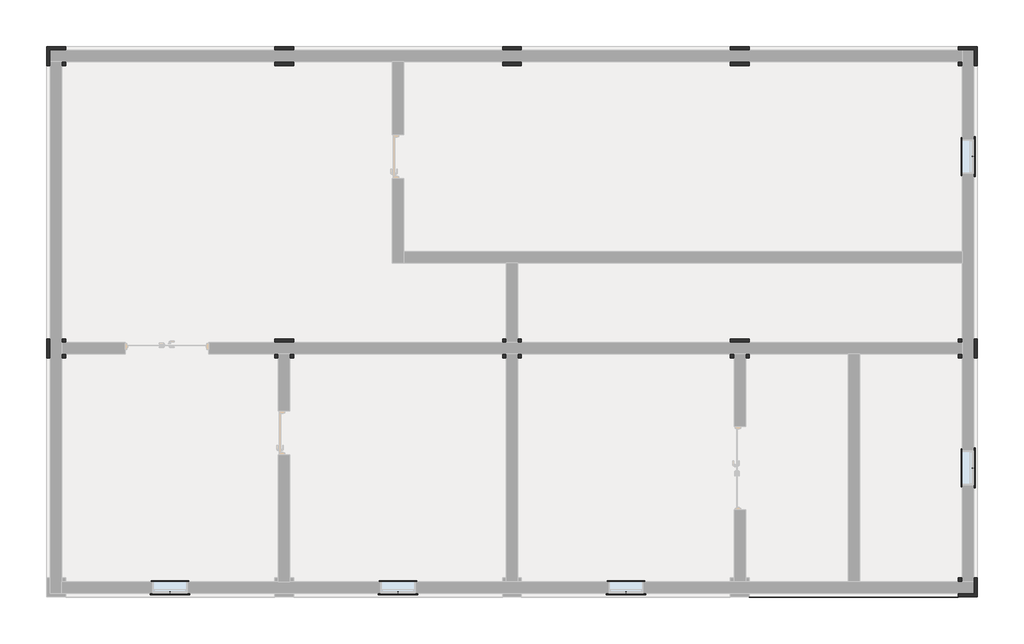
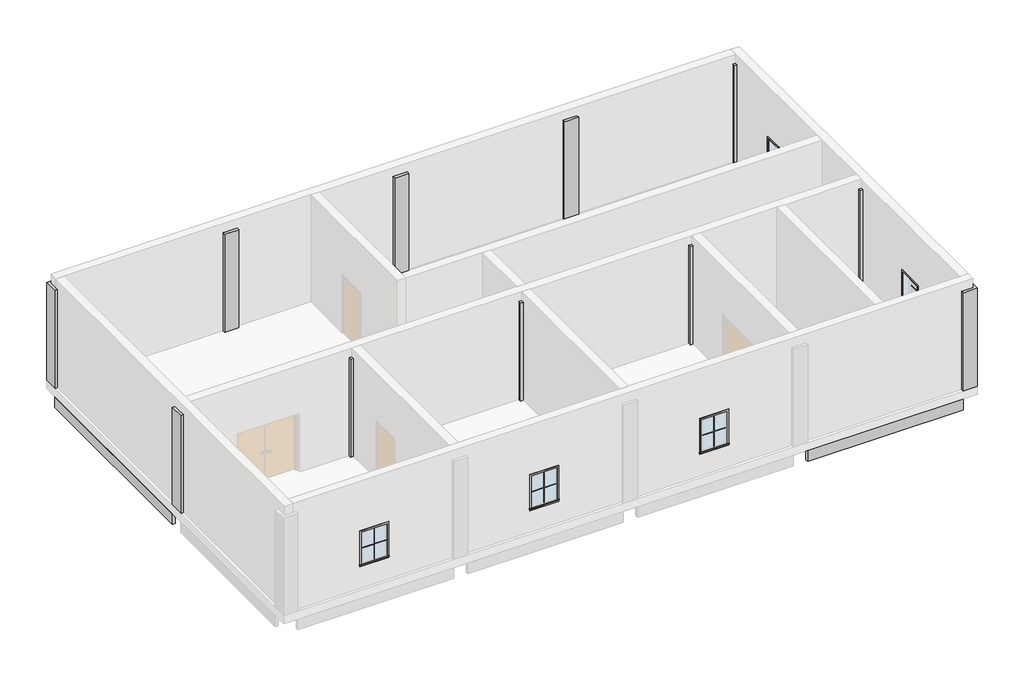
# One storey, part 2 of 2: 16 beams, 15 proxies, 11 columns.
"""IFC4 building model written with IfcOpenShell, lengths in millimetres."""

import ifcopenshell
import ifcopenshell.guid

model = None  # the IFC model being written
_history = None  # IfcOwnerHistory: only IFC2X3 demands one
_inside = {}  # id of a spatial element -> (the spatial element, [elements in it])
_under = {}  # id of a project, library or spatial element -> (it, [spatial elements below it])
_declared = {}  # id of a project -> (the project, [libraries it declares])
_typed = {}  # id of a type object -> (the type object, [elements of that type])
_made_of = {}  # id of a material, layer set ... -> (it, [elements and type objects made of it])


def new_model(schema):
    """Start an empty IFC model of exactly this schema.

    Asked for "IFC4X3", IfcOpenShell would pick the latest addendum, in which some entities
    have other attributes; the version numbers below select the first issue.
    IFC2X3 requires an IfcOwnerHistory on every rooted entity: one is made here for all.
    """
    global model, _history
    if schema == "IFC4X3":
        model = ifcopenshell.file(schema_version=(4, 3, 0, 0))
    else:
        model = ifcopenshell.file(schema=schema)
    _inside.clear()
    _under.clear()
    _declared.clear()
    _typed.clear()
    _made_of.clear()
    _history = None
    if model.schema == "IFC2X3":
        org = make("IfcOrganization", Name="unknown")
        user = make(
            "IfcPersonAndOrganization",
            ThePerson=make("IfcPerson", FamilyName="unknown"),
            TheOrganization=org,
        )
        app = make(
            "IfcApplication",
            ApplicationDeveloper=org,
            Version="unknown",
            ApplicationFullName="unknown",
            ApplicationIdentifier="unknown",
        )
        _history = make(
            "IfcOwnerHistory",
            OwningUser=user,
            OwningApplication=app,
            ChangeAction="ADDED",
            CreationDate=0,
        )
    return model


def make(cls, **values):
    """One entity of the class cls with the attributes given. An attribute that is None is left unset."""
    return model.create_entity(
        cls, **{name: value for name, value in values.items() if value is not None}
    )


def rooted(cls, **values):
    """An entity with a GlobalId (a new one), such as an element, a storey or a relation."""
    return make(cls, GlobalId=ifcopenshell.guid.new(), OwnerHistory=_history, **values)


def si_unit(unit_type, name, prefix=None):
    """IfcSIUnit, for example si_unit("LENGTHUNIT", "METRE", prefix="MILLI")."""
    return make("IfcSIUnit", UnitType=unit_type, Prefix=prefix, Name=name)


def assignment(units):
    """IfcUnitAssignment: the units of a project."""
    return None if units is None else make("IfcUnitAssignment", Units=units)


def point(xyz):
    """IfcCartesianPoint."""
    return None if xyz is None else make("IfcCartesianPoint", Coordinates=xyz)


def direction(xyz):
    """IfcDirection."""
    return None if xyz is None else make("IfcDirection", DirectionRatios=xyz)


def frame(location, z_axis=None, x_axis=None):
    """IfcAxis2Placement3D, a coordinate frame: its origin and axes. An axis left out is left unset."""
    return make(
        "IfcAxis2Placement3D",
        Location=point(location),
        Axis=direction(z_axis),
        RefDirection=direction(x_axis),
    )


def origin():
    """The frame at (0, 0, 0) with its axes left unset."""
    return frame((0.0, 0.0, 0.0))


def origin_with_axes():
    """The frame at (0, 0, 0) with the z axis (0, 0, 1) and the x axis (1, 0, 0) written out."""
    return frame((0.0, 0.0, 0.0), z_axis=(0.0, 0.0, 1.0), x_axis=(1.0, 0.0, 0.0))


def place(relative_to, where):
    """IfcLocalPlacement: puts the frame where relative to a parent placement (None: the world)."""
    return make(
        "IfcLocalPlacement", PlacementRelTo=relative_to, RelativePlacement=where
    )


def context(
    kind, dimensions, precision=None, world=None, true_north=None, identifier=None
):
    """IfcGeometricRepresentationContext, for example the 3D "Model" context."""
    return make(
        "IfcGeometricRepresentationContext",
        ContextIdentifier=identifier,
        ContextType=kind,
        CoordinateSpaceDimension=dimensions,
        Precision=precision,
        WorldCoordinateSystem=world,
        TrueNorth=true_north,
    )


def project(units=None, contexts=None):
    """IfcProject with its units and contexts."""
    return rooted(
        "IfcProject",
        Name="project",
        RepresentationContexts=contexts,
        UnitsInContext=assignment(units),
    )


def spatial(cls, under=None, at=None, **own):
    """A site, building, storey or space (cls), placed at a placement, below another one or the project."""
    s = rooted(cls, ObjectPlacement=at, **own)
    if under is not None:
        _under.setdefault(under.id(), (under, []))[1].append(s)
    return s


def polyline(points):
    """IfcPolyline through the points."""
    return make("IfcPolyline", Points=[point(p) for p in points])


def outline(outer, holes=None, kind="AREA"):
    """IfcArbitraryClosedProfileDef: a profile drawn as a closed curve; with holes, ...WithVoids."""
    if holes is None:
        return make("IfcArbitraryClosedProfileDef", ProfileType=kind, OuterCurve=outer)
    return make(
        "IfcArbitraryProfileDefWithVoids",
        ProfileType=kind,
        OuterCurve=outer,
        InnerCurves=holes,
    )


def extrude(swept, where, along, depth):
    """IfcExtrudedAreaSolid: the profile swept, set in the frame where, extruded along a direction by depth."""
    return make(
        "IfcExtrudedAreaSolid",
        SweptArea=swept,
        Position=where,
        ExtrudedDirection=direction(along),
        Depth=depth,
    )


def faces_of(points, faces, orient=None, outer=None):
    """IfcFace entities. A face is a list of loops; a loop is a list of indices into points, from 0.

    orient and outer hold one flag for each loop. By default every Orientation is true, the
    first loop of a face is its IfcFaceOuterBound and the others are IfcFaceBound.
    """
    made = []
    for i, loops in enumerate(faces):
        bounds = []
        for j, loop in enumerate(loops):
            is_outer = j == 0 if outer is None else outer[i][j]
            bounds.append(
                make(
                    "IfcFaceOuterBound" if is_outer else "IfcFaceBound",
                    Bound=make("IfcPolyLoop", Polygon=[points[k] for k in loop]),
                    Orientation=True if orient is None else orient[i][j],
                )
            )
        made.append(make("IfcFace", Bounds=bounds))
    return made


def faceted_brep(points, faces, orient=None, outer=None, voids=None):
    """IfcFacetedBrep: a solid bounded by flat faces; with voids (closed shells), ...WithVoids."""
    shared = [point(p) for p in points]
    hull = make("IfcClosedShell", CfsFaces=faces_of(shared, faces, orient, outer))
    if voids is None:
        return make("IfcFacetedBrep", Outer=hull)
    return make(
        "IfcFacetedBrepWithVoids",
        Outer=hull,
        Voids=[
            make(cls, CfsFaces=faces_of(shared, fs, o, b)) for cls, fs, o, b in voids
        ],
    )


def shape(context_of_items, identifier, shape_type, items):
    """IfcShapeRepresentation: the items that make up one representation, for example the "Body"."""
    return make(
        "IfcShapeRepresentation",
        ContextOfItems=context_of_items,
        RepresentationIdentifier=identifier,
        RepresentationType=shape_type,
        Items=items,
    )


def source(mapping_origin, context_of_items, identifier, shape_type, items):
    """IfcRepresentationMap: a shape defined once, which mapped items show again and again."""
    return make(
        "IfcRepresentationMap",
        MappingOrigin=mapping_origin,
        MappedRepresentation=shape(context_of_items, identifier, shape_type, items),
    )


def transform(
    local_origin,
    x_axis=None,
    y_axis=None,
    z_axis=None,
    scale=None,
    scale2=None,
    scale3=None,
    uniform=True,
):
    """IfcCartesianTransformationOperator3D, or its non-uniform kind. x_axis, y_axis, z_axis: its Axis1, 2, 3."""
    if uniform:
        return make(
            "IfcCartesianTransformationOperator3D",
            Axis1=direction(x_axis),
            Axis2=direction(y_axis),
            LocalOrigin=point(local_origin),
            Scale=scale,
            Axis3=direction(z_axis),
        )
    return make(
        "IfcCartesianTransformationOperator3DnonUniform",
        Axis1=direction(x_axis),
        Axis2=direction(y_axis),
        LocalOrigin=point(local_origin),
        Scale=scale,
        Axis3=direction(z_axis),
        Scale2=scale2,
        Scale3=scale3,
    )


def mapped(mapping_source, mapping_target):
    """IfcMappedItem: shows the shape of a source again, moved by a transform."""
    return make(
        "IfcMappedItem", MappingSource=mapping_source, MappingTarget=mapping_target
    )


def made_of(thing, what):
    """Note that an element or type object is made of a material, layer set ...; save() writes the relation."""
    if what is not None:
        _made_of.setdefault(what.id(), (what, []))[1].append(thing)
    return thing


def element(
    cls,
    number,
    at=None,
    inside=None,
    cuts=None,
    type_object=None,
    material=None,
    context=None,
    identifier="Body",
    shape_type=None,
    held_by="IfcProductDefinitionShape",
    body=None,
    shapes=None,
    **own,
):
    """One element of the class cls, such as IfcWall. Its Tag is "e" and its number.

    at: its placement. inside: the storey or other place that contains it. cuts: it is an
    opening in that element (IfcRelVoidsElement). A single representation is given by context,
    identifier, shape_type and body (its items); several are given by shapes. held_by: the class
    of the entity that holds the representations. save() writes the other relations.
    """
    e = rooted(cls, Tag="e%d" % number, ObjectPlacement=at, **own)
    if body is not None:
        shapes = [shape(context, identifier, shape_type, body)]
    if shapes is not None:
        e.Representation = make(held_by, Representations=shapes)
    if inside is not None:
        _inside.setdefault(inside.id(), (inside, []))[1].append(e)
    if cuts is not None:
        rooted(
            "IfcRelVoidsElement", RelatingBuildingElement=cuts, RelatedOpeningElement=e
        )
    if type_object is not None:
        _typed.setdefault(type_object.id(), (type_object, []))[1].append(e)
    return made_of(e, material)


def aggregate(whole, parts):
    """IfcRelAggregates: a whole, such as a stair, and the parts it consists of."""
    return rooted("IfcRelAggregates", RelatingObject=whole, RelatedObjects=parts)


def save(model, path):
    """Write the relations noted so far, then the file.

    IfcRelAggregates (storeys below a building ...), IfcRelContainedInSpatialStructure (elements
    in a storey), IfcRelDefinesByType, IfcRelAssociatesMaterial and IfcRelDeclares: one each for
    every whole, place, type object, material and project.
    """
    for whole, parts in _under.values():
        aggregate(whole, parts)
    for where, things in _inside.values():
        rooted(
            "IfcRelContainedInSpatialStructure",
            RelatedElements=things,
            RelatingStructure=where,
        )
    for kind, things in _typed.values():
        rooted("IfcRelDefinesByType", RelatedObjects=things, RelatingType=kind)
    for what, things in _made_of.values():
        rooted("IfcRelAssociatesMaterial", RelatedObjects=things, RelatingMaterial=what)
    for by, libraries in _declared.values():
        rooted("IfcRelDeclares", RelatingContext=by, RelatedDefinitions=libraries)
    model.write(path)


def m_muntin_pattern_2x2_m_muntin_pattern_2x2_ad852c99(model_context):
    return source(origin(), model_context, "Body", "SweptSolid", [
        extrude(outline(polyline([(568.25, -6.35), (568.25, -411.9), (555.55, -411.9), (555.55, -6.35), (0.0, -6.35), (0.0, 6.35), (555.55, 6.35), (555.55, 411.9), (568.25, 411.9), (568.25, 6.35), (1123.8, 6.35), (1123.8, -6.35), (568.25, -6.35)])), frame((0.0, -22.225, 0.0), z_axis=(0.0, 1.0, 0.0), x_axis=(0.0, 0.0, 1.0)), (0.0, 0.0, 1.0), 12.7),
        extrude(outline(polyline([(568.25, -6.35), (568.25, -411.9), (555.55, -411.9), (555.55, -6.35), (0.0, -6.35), (0.0, 6.35), (555.55, 6.35), (555.55, 411.9), (568.25, 411.9), (568.25, 6.35), (1123.8, 6.35), (1123.8, -6.35), (568.25, -6.35)])), frame((0.0, 9.525, 0.0), z_axis=(0.0, 1.0, 0.0), x_axis=(0.0, 0.0, 1.0)), (0.0, 0.0, 1.0), 12.7),
    ])


def m_trim_window_exterior_flat_with_sill_71544b40(model_context):
    return source(origin(), model_context, "Body", "SweptSolid", [
        extrude(outline(polyline([(510.0, -1220.4323709), (510.0, -1280.4323709), (-510.0, -1280.4323709), (-510.0, -1220.4323709), (510.0, -1220.4323709)])), origin_with_axes(), (0.0, 0.0, 1.0), 19.05),
        extrude(outline(polyline([(-1230.0, 38.1), (-1202.4580645, 38.1), (-1200.0, 19.05), (-1200.0, 0.0), (-1220.4323709, 0.0), (-1220.4323709, 19.05), (-1230.0, 19.05), (-1230.0, 38.1)])), frame((-522.7, 0.0, 0.0), z_axis=(1.0, 0.0, 0.0), x_axis=(0.0, 1.0, 0.0)), (0.0, 0.0, 1.0), 1045.4),
        extrude(outline(polyline([(-510.0, 60.0), (510.0, 60.0), (510.0, -1200.0), (450.0, -1200.0), (450.0, 0.0), (-450.0, 0.0), (-450.0, -1200.0), (-510.0, -1200.0), (-510.0, 60.0)])), origin_with_axes(), (0.0, 0.0, 1.0), 19.05),
    ])


def m_trim_window_interior_flat_picture_frame_24fe8ef8(model_context):
    return source(origin(), model_context, "Body", "SweptSolid", [
        extrude(outline(polyline([(497.3, 47.3), (497.3, -1247.3), (-497.3, -1247.3), (-497.3, 47.3), (497.3, 47.3)]), holes=[polyline([(437.3, -12.7), (-437.3, -12.7), (-437.3, -1187.3), (437.3, -1187.3), (437.3, -12.7)])]), origin_with_axes(), (0.0, 0.0, 1.0), 30.0),
    ])


model = new_model("IFC4")

# Units and contexts
model_context = context("Model", 3, world=origin())
ifc_project = project(units=[si_unit("LENGTHUNIT", "METRE", prefix="MILLI")], contexts=[model_context])

# Site, building, storey
site = spatial("IfcSite", under=ifc_project)
building = spatial("IfcBuilding", under=site)
storey = spatial("IfcBuildingStorey", under=building, Name="2nd FL GL+6,200", Elevation=6000.0)

# Beams
placement = place(None, origin())
element("IfcBeam", 1, ObjectType="RC Beam_Rectangular : 350 x 700mm", at=placement, inside=storey, context=model_context, shape_type="SweptSolid", body=[
    extrude(outline(polyline([(-18945.7273237, 9185.9763125), (-18845.7273237, 9185.9763125), (-18845.7273237, 1985.9763125), (-18945.7273237, 1985.9763125), (-18945.7273237, 9185.9763125)])), frame((0.0, 0.0, 5300.0), z_axis=(0.0, 0.0, 1.0), x_axis=(1.0, 0.0, 0.0)), (0.0, 0.0, 1.0), 400.0),
])
element("IfcBeam", 2, ObjectType="RC Beam_Rectangular : 350 x 700mm", at=placement, inside=storey, context=model_context, shape_type="SweptSolid", body=[
    extrude(outline(polyline([(-12870.7273237, 9185.9763125), (-12520.7273237, 9185.9763125), (-12520.7273237, 1985.9763125), (-12870.7273237, 1985.9763125), (-12870.7273237, 9185.9763125)])), frame((0.0, 0.0, 5300.0), z_axis=(0.0, 0.0, 1.0), x_axis=(1.0, 0.0, 0.0)), (0.0, 0.0, 1.0), 400.0),
])
element("IfcBeam", 3, ObjectType="RC Beam_Rectangular : 350 x 700mm", at=placement, inside=storey, context=model_context, shape_type="SweptSolid", body=[
    extrude(outline(polyline([(-6870.7273237, 9185.9763125), (-6520.7273237, 9185.9763125), (-6520.7273237, 1985.9763125), (-6870.7273237, 1985.9763125), (-6870.7273237, 9185.9763125)])), frame((0.0, 0.0, 5300.0), z_axis=(0.0, 0.0, 1.0), x_axis=(1.0, 0.0, 0.0)), (0.0, 0.0, 1.0), 400.0),
])
element("IfcBeam", 4, ObjectType="RC Beam_Rectangular : 350 x 700mm", at=placement, inside=storey, context=model_context, shape_type="SweptSolid", body=[
    extrude(outline(polyline([(-520.7273237, 1485.9763125), (-520.7273237, -4314.0236875), (-545.7273237, -4314.0236875), (-545.7273237, 1485.9763125), (-520.7273237, 1485.9763125)])), frame((0.0, 0.0, 5300.0), z_axis=(0.0, 0.0, 1.0), x_axis=(1.0, 0.0, 0.0)), (0.0, 0.0, 1.0), 400.0),
    extrude(outline(polyline([(-870.7273237, -4314.0236875), (-870.7273237, 1485.9763125), (-845.7273237, 1485.9763125), (-845.7273237, -4314.0236875), (-870.7273237, -4314.0236875)])), frame((0.0, 0.0, 5300.0), z_axis=(0.0, 0.0, 1.0), x_axis=(1.0, 0.0, 0.0)), (0.0, 0.0, 1.0), 400.0),
])
element("IfcBeam", 5, ObjectType="RC Beam_Rectangular : 350 x 700mm", at=placement, inside=storey, context=model_context, shape_type="SweptSolid", body=[
    extrude(outline(polyline([(-870.7273237, 9185.9763125), (-520.7273237, 9185.9763125), (-520.7273237, 1985.9763125), (-870.7273237, 1985.9763125), (-870.7273237, 9185.9763125)])), frame((0.0, 0.0, 5300.0), z_axis=(0.0, 0.0, 1.0), x_axis=(1.0, 0.0, 0.0)), (0.0, 0.0, 1.0), 400.0),
])
element("IfcBeam", 6, ObjectType="RC Beam_Rectangular : 350 x 700mm", at=placement, inside=storey, context=model_context, shape_type="SweptSolid", body=[
    extrude(outline(polyline([(5554.2726763, 1485.9763125), (5554.2726763, -4314.0236875), (5454.2726763, -4314.0236875), (5454.2726763, 1485.9763125), (5554.2726763, 1485.9763125)])), frame((0.0, 0.0, 5300.0), z_axis=(0.0, 0.0, 1.0), x_axis=(1.0, 0.0, 0.0)), (0.0, 0.0, 1.0), 400.0),
])
element("IfcBeam", 7, ObjectType="RC Beam_Rectangular : 350 x 700mm", at=placement, inside=storey, context=model_context, shape_type="SweptSolid", body=[
    extrude(outline(polyline([(5554.2726763, 9185.9763125), (5554.2726763, 1998.6763125), (5454.2726763, 1998.6763125), (5454.2726763, 9185.9763125), (5554.2726763, 9185.9763125)])), frame((0.0, 0.0, 5300.0), z_axis=(0.0, 0.0, 1.0), x_axis=(1.0, 0.0, 0.0)), (0.0, 0.0, 1.0), 400.0),
])
element("IfcBeam", 8, ObjectType="RC Beam_Rectangular : 350 x 700mm", at=placement, inside=storey, context=model_context, shape_type="SweptSolid", body=[
    extrude(outline(polyline([(-18445.7273237, 9685.9763125), (-12945.7273237, 9685.9763125), (-12945.7273237, 9585.9763125), (-18445.7273237, 9585.9763125), (-18445.7273237, 9685.9763125)])), frame((0.0, 0.0, 5300.0), z_axis=(0.0, 0.0, 1.0), x_axis=(1.0, 0.0, 0.0)), (0.0, 0.0, 1.0), 400.0),
])
element("IfcBeam", 9, ObjectType="RC Beam_Rectangular : 350 x 700mm", at=placement, inside=storey, context=model_context, shape_type="SweptSolid", body=[
    extrude(outline(polyline([(-12433.0273237, 9685.9763125), (-6945.7273237, 9685.9763125), (-6945.7273237, 9585.9763125), (-12433.0273237, 9585.9763125), (-12433.0273237, 9685.9763125)])), frame((0.0, 0.0, 5300.0), z_axis=(0.0, 0.0, 1.0), x_axis=(1.0, 0.0, 0.0)), (0.0, 0.0, 1.0), 400.0),
])
element("IfcBeam", 10, ObjectType="RC Beam_Rectangular : 350 x 700mm", at=placement, inside=storey, context=model_context, shape_type="SweptSolid", body=[
    extrude(outline(polyline([(-6433.0273237, 9685.9763125), (-945.7273237, 9685.9763125), (-945.7273237, 9585.9763125), (-6433.0273237, 9585.9763125), (-6433.0273237, 9685.9763125)])), frame((0.0, 0.0, 5300.0), z_axis=(0.0, 0.0, 1.0), x_axis=(1.0, 0.0, 0.0)), (0.0, 0.0, 1.0), 400.0),
])
element("IfcBeam", 11, ObjectType="RC Beam_Rectangular : 350 x 700mm", at=placement, inside=storey, context=model_context, shape_type="SweptSolid", body=[
    extrude(outline(polyline([(-433.0273237, 9685.9763125), (5054.2726763, 9685.9763125), (5054.2726763, 9585.9763125), (-433.0273237, 9585.9763125), (-433.0273237, 9685.9763125)])), frame((0.0, 0.0, 5300.0), z_axis=(0.0, 0.0, 1.0), x_axis=(1.0, 0.0, 0.0)), (0.0, 0.0, 1.0), 400.0),
])
element("IfcBeam", 12, ObjectType="RC Beam_Rectangular : 350 x 700mm", at=placement, inside=storey, context=model_context, shape_type="SweptSolid", body=[
    extrude(outline(polyline([(-12945.7273237, 1560.9763125), (-18445.7273237, 1560.9763125), (-18445.7273237, 1585.9763125), (-12945.7273237, 1585.9763125), (-12945.7273237, 1560.9763125)])), frame((0.0, 0.0, 5300.0), z_axis=(0.0, 0.0, 1.0), x_axis=(1.0, 0.0, 0.0)), (0.0, 0.0, 1.0), 400.0),
    extrude(outline(polyline([(-18445.7273237, 1910.9763125), (-12945.7273237, 1910.9763125), (-12945.7273237, 1885.9763125), (-18445.7273237, 1885.9763125), (-18445.7273237, 1910.9763125)])), frame((0.0, 0.0, 5300.0), z_axis=(0.0, 0.0, 1.0), x_axis=(1.0, 0.0, 0.0)), (0.0, 0.0, 1.0), 400.0),
])
element("IfcBeam", 13, ObjectType="RC Beam_Rectangular : 350 x 700mm", at=placement, inside=storey, context=model_context, shape_type="SweptSolid", body=[
    extrude(outline(polyline([(-6945.7273237, 1585.9763125), (-6945.7273237, 1560.9763125), (-12445.7273237, 1560.9763125), (-12445.7273237, 1585.9763125), (-6945.7273237, 1585.9763125)])), frame((0.0, 0.0, 5300.0), z_axis=(0.0, 0.0, 1.0), x_axis=(1.0, 0.0, 0.0)), (0.0, 0.0, 1.0), 400.0),
    extrude(outline(polyline([(-6945.7273237, 1910.9763125), (-6945.7273237, 1885.9763125), (-12445.7273237, 1885.9763125), (-12445.7273237, 1910.9763125), (-6945.7273237, 1910.9763125)])), frame((0.0, 0.0, 5300.0), z_axis=(0.0, 0.0, 1.0), x_axis=(1.0, 0.0, 0.0)), (0.0, 0.0, 1.0), 400.0),
])
element("IfcBeam", 14, ObjectType="RC Beam_Rectangular : 350 x 700mm", at=placement, inside=storey, context=model_context, shape_type="SweptSolid", body=[
    extrude(outline(polyline([(-945.7273237, 1585.9763125), (-945.7273237, 1560.9763125), (-6445.7273237, 1560.9763125), (-6445.7273237, 1585.9763125), (-945.7273237, 1585.9763125)])), frame((0.0, 0.0, 5300.0), z_axis=(0.0, 0.0, 1.0), x_axis=(1.0, 0.0, 0.0)), (0.0, 0.0, 1.0), 400.0),
    extrude(outline(polyline([(-945.7273237, 1910.9763125), (-945.7273237, 1885.9763125), (-6445.7273237, 1885.9763125), (-6445.7273237, 1910.9763125), (-945.7273237, 1910.9763125)])), frame((0.0, 0.0, 5300.0), z_axis=(0.0, 0.0, 1.0), x_axis=(1.0, 0.0, 0.0)), (0.0, 0.0, 1.0), 400.0),
])
element("IfcBeam", 15, ObjectType="RC Beam_Rectangular : 350 x 700mm", at=placement, inside=storey, context=model_context, shape_type="SweptSolid", body=[
    extrude(outline(polyline([(2154.2726763, 1585.9763125), (2154.2726763, 1560.9763125), (-445.7273237, 1560.9763125), (-445.7273237, 1585.9763125), (2154.2726763, 1585.9763125)])), frame((0.0, 0.0, 5300.0), z_axis=(0.0, 0.0, 1.0), x_axis=(1.0, 0.0, 0.0)), (0.0, 0.0, 1.0), 400.0),
    extrude(outline(polyline([(5054.2726763, 1910.9763125), (5054.2726763, 1885.9763125), (-445.7273237, 1885.9763125), (-445.7273237, 1910.9763125), (5054.2726763, 1910.9763125)])), frame((0.0, 0.0, 5300.0), z_axis=(0.0, 0.0, 1.0), x_axis=(1.0, 0.0, 0.0)), (0.0, 0.0, 1.0), 400.0),
    extrude(outline(polyline([(5054.2726763, 1585.9763125), (5054.2726763, 1560.9763125), (2454.2726763, 1560.9763125), (2454.2726763, 1585.9763125), (5054.2726763, 1585.9763125)])), frame((0.0, 0.0, 5300.0), z_axis=(0.0, 0.0, 1.0), x_axis=(1.0, 0.0, 0.0)), (0.0, 0.0, 1.0), 400.0),
])
element("IfcBeam", 16, ObjectType="RC Beam_Rectangular : 350 x 700mm", at=placement, inside=storey, context=model_context, shape_type="SweptSolid", body=[
    extrude(outline(polyline([(5054.2726763, -4714.0236875), (5054.2726763, -4814.0236875), (-445.7273237, -4814.0236875), (-445.7273237, -4714.0236875), (5054.2726763, -4714.0236875)])), frame((0.0, 0.0, 5300.0), z_axis=(0.0, 0.0, 1.0), x_axis=(1.0, 0.0, 0.0)), (0.0, 0.0, 1.0), 400.0),
])

# Proxies
m_muntin_pattern_2x2_m_muntin_pattern_2x2_shape = m_muntin_pattern_2x2_m_muntin_pattern_2x2_ad852c99(model_context)
element("IfcBuildingElementProxy", 17, Name="M_Muntin Pattern_2x2 : M_Muntin Pattern_2x2", ObjectType="M_Muntin Pattern_2x2 : M_Muntin Pattern_2x2", at=placement, inside=storey, context=model_context, shape_type="MappedRepresentation", body=[
    mapped(m_muntin_pattern_2x2_m_muntin_pattern_2x2_shape, transform((5444.7476763, 6785.9763125, 6938.1), x_axis=(0.0, 1.0, 0.0), y_axis=(-1.0, 0.0, 0.0), z_axis=(0.0, 0.0, 1.0))),
])
element("IfcBuildingElementProxy", 18, Name="M_Muntin Pattern_2x2 : M_Muntin Pattern_2x2", ObjectType="M_Muntin Pattern_2x2 : M_Muntin Pattern_2x2", at=placement, inside=storey, context=model_context, shape_type="MappedRepresentation", body=[
    mapped(m_muntin_pattern_2x2_m_muntin_pattern_2x2_shape, transform((5444.7476763, -1414.0236875, 6938.1), x_axis=(0.0, 1.0, 0.0), y_axis=(-1.0, 0.0, 0.0), z_axis=(0.0, 0.0, 1.0))),
])
element("IfcBuildingElementProxy", 19, Name="M_Muntin Pattern_2x2 : M_Muntin Pattern_2x2", ObjectType="M_Muntin Pattern_2x2 : M_Muntin Pattern_2x2", at=placement, inside=storey, context=model_context, shape_type="MappedRepresentation", body=[
    mapped(m_muntin_pattern_2x2_m_muntin_pattern_2x2_shape, transform((-15695.7273237, -4704.4986875, 6938.1), x_axis=(1.0, 0.0, 0.0), y_axis=(0.0, 1.0, 0.0), z_axis=(0.0, 0.0, 1.0))),
])
element("IfcBuildingElementProxy", 20, Name="M_Muntin Pattern_2x2 : M_Muntin Pattern_2x2", ObjectType="M_Muntin Pattern_2x2 : M_Muntin Pattern_2x2", at=placement, inside=storey, context=model_context, shape_type="MappedRepresentation", body=[
    mapped(m_muntin_pattern_2x2_m_muntin_pattern_2x2_shape, transform((-9695.7273237, -4704.4986875, 6938.1), x_axis=(1.0, 0.0, 0.0), y_axis=(0.0, 1.0, 0.0), z_axis=(0.0, 0.0, 1.0))),
])
element("IfcBuildingElementProxy", 21, Name="M_Muntin Pattern_2x2 : M_Muntin Pattern_2x2", ObjectType="M_Muntin Pattern_2x2 : M_Muntin Pattern_2x2", at=placement, inside=storey, context=model_context, shape_type="MappedRepresentation", body=[
    mapped(m_muntin_pattern_2x2_m_muntin_pattern_2x2_shape, transform((-3695.7273237, -4704.4986875, 6938.1), x_axis=(1.0, 0.0, 0.0), y_axis=(0.0, 1.0, 0.0), z_axis=(0.0, 0.0, 1.0))),
])
m_trim_window_exterior_flat_with_sill_shape = m_trim_window_exterior_flat_with_sill_71544b40(model_context)
element("IfcBuildingElementProxy", 22, Name="M_Trim-Window-Exterior-Flat : with Sill", ObjectType="M_Trim-Window-Exterior-Flat : with Sill", at=placement, inside=storey, context=model_context, shape_type="MappedRepresentation", body=[
    mapped(m_trim_window_exterior_flat_with_sill_shape, transform((5454.2726763, 6785.9763125, 8100.0), x_axis=(0.0, 1.0, 0.0), y_axis=(0.0, 0.0, 1.0), z_axis=(1.0, 0.0, 0.0))),
])
element("IfcBuildingElementProxy", 23, Name="M_Trim-Window-Exterior-Flat : with Sill", ObjectType="M_Trim-Window-Exterior-Flat : with Sill", at=placement, inside=storey, context=model_context, shape_type="MappedRepresentation", body=[
    mapped(m_trim_window_exterior_flat_with_sill_shape, transform((5454.2726763, -1414.0236875, 8100.0), x_axis=(0.0, 1.0, 0.0), y_axis=(0.0, 0.0, 1.0), z_axis=(1.0, 0.0, 0.0))),
])
element("IfcBuildingElementProxy", 24, Name="M_Trim-Window-Exterior-Flat : with Sill", ObjectType="M_Trim-Window-Exterior-Flat : with Sill", at=placement, inside=storey, context=model_context, shape_type="MappedRepresentation", body=[
    mapped(m_trim_window_exterior_flat_with_sill_shape, transform((-15695.7273237, -4714.0236875, 8100.0), x_axis=(1.0, 0.0, 0.0), y_axis=(0.0, 0.0, 1.0), z_axis=(0.0, -1.0, 0.0))),
])
element("IfcBuildingElementProxy", 25, Name="M_Trim-Window-Exterior-Flat : with Sill", ObjectType="M_Trim-Window-Exterior-Flat : with Sill", at=placement, inside=storey, context=model_context, shape_type="MappedRepresentation", body=[
    mapped(m_trim_window_exterior_flat_with_sill_shape, transform((-9695.7273237, -4714.0236875, 8100.0), x_axis=(1.0, 0.0, 0.0), y_axis=(0.0, 0.0, 1.0), z_axis=(0.0, -1.0, 0.0))),
])
element("IfcBuildingElementProxy", 26, Name="M_Trim-Window-Exterior-Flat : with Sill", ObjectType="M_Trim-Window-Exterior-Flat : with Sill", at=placement, inside=storey, context=model_context, shape_type="MappedRepresentation", body=[
    mapped(m_trim_window_exterior_flat_with_sill_shape, transform((-3695.7273237, -4714.0236875, 8100.0), x_axis=(1.0, 0.0, 0.0), y_axis=(0.0, 0.0, 1.0), z_axis=(0.0, -1.0, 0.0))),
])
m_trim_window_interior_flat_picture_frame_shape = m_trim_window_interior_flat_picture_frame_24fe8ef8(model_context)
element("IfcBuildingElementProxy", 27, Name="M_Trim-Window-Interior-Flat : Picture Frame", ObjectType="M_Trim-Window-Interior-Flat : Picture Frame", at=placement, inside=storey, context=model_context, shape_type="MappedRepresentation", body=[
    mapped(m_trim_window_interior_flat_picture_frame_shape, transform((5154.2726763, 6785.9763125, 8100.0), x_axis=(0.0, -1.0, 0.0), y_axis=(0.0, 0.0, 1.0), z_axis=(-1.0, 0.0, 0.0))),
])
element("IfcBuildingElementProxy", 28, Name="M_Trim-Window-Interior-Flat : Picture Frame", ObjectType="M_Trim-Window-Interior-Flat : Picture Frame", at=placement, inside=storey, context=model_context, shape_type="MappedRepresentation", body=[
    mapped(m_trim_window_interior_flat_picture_frame_shape, transform((5154.2726763, -1414.0236875, 8100.0), x_axis=(0.0, -1.0, 0.0), y_axis=(0.0, 0.0, 1.0), z_axis=(-1.0, 0.0, 0.0))),
])
element("IfcBuildingElementProxy", 29, Name="M_Trim-Window-Interior-Flat : Picture Frame", ObjectType="M_Trim-Window-Interior-Flat : Picture Frame", at=placement, inside=storey, context=model_context, shape_type="MappedRepresentation", body=[
    mapped(m_trim_window_interior_flat_picture_frame_shape, transform((-15695.7273237, -4414.0236875, 8100.0), x_axis=(-1.0, 0.0, 0.0), y_axis=(0.0, 0.0, 1.0), z_axis=(0.0, 1.0, 0.0))),
])
element("IfcBuildingElementProxy", 30, Name="M_Trim-Window-Interior-Flat : Picture Frame", ObjectType="M_Trim-Window-Interior-Flat : Picture Frame", at=placement, inside=storey, context=model_context, shape_type="MappedRepresentation", body=[
    mapped(m_trim_window_interior_flat_picture_frame_shape, transform((-9695.7273237, -4414.0236875, 8100.0), x_axis=(-1.0, 0.0, 0.0), y_axis=(0.0, 0.0, 1.0), z_axis=(0.0, 1.0, 0.0))),
])
element("IfcBuildingElementProxy", 31, Name="M_Trim-Window-Interior-Flat : Picture Frame", ObjectType="M_Trim-Window-Interior-Flat : Picture Frame", at=placement, inside=storey, context=model_context, shape_type="MappedRepresentation", body=[
    mapped(m_trim_window_interior_flat_picture_frame_shape, transform((-3695.7273237, -4414.0236875, 8100.0), x_axis=(-1.0, 0.0, 0.0), y_axis=(0.0, 0.0, 1.0), z_axis=(0.0, 1.0, 0.0))),
])

# Columns
element("IfcColumn", 32, ObjectType="RC_Column_Rectangular : 500 x 500mm", at=placement, inside=storey, context=model_context, shape_type="Brep", body=[
    faceted_brep([(-18945.7273237, 9185.9763125, 6000.0), (-18945.7273237, 9685.9763125, 6000.0), (-18445.7273237, 9685.9763125, 6000.0), (-18445.7273237, 9585.9763125, 6000.0), (-18845.7273237, 9585.9763125, 6000.0), (-18845.7273237, 9285.9763125, 6000.0), (-18845.7273237, 9185.9763125, 6000.0), (-18945.7273237, 9685.9763125, 9667.0), (-18445.7273237, 9685.9763125, 9667.0), (-18445.7273237, 9685.9763125, 9300.0), (-18945.7273237, 9185.9763125, 9300.0), (-18945.7273237, 9185.9763125, 9667.0), (-18845.7273237, 9185.9763125, 9300.0), (-18845.7273237, 9185.9763125, 9667.0), (-18445.7273237, 9585.9763125, 9667.0), (-18445.7273237, 9585.9763125, 9300.0), (-18845.7273237, 9585.9763125, 9667.0)], [[[0, 1, 2, 3, 4, 5, 6]], [[2, 1, 7, 8, 9]], [[1, 0, 10, 11, 7]], [[11, 10, 0, 6, 12, 13]], [[2, 9, 8, 14, 15, 3]], [[8, 7, 11, 13, 16, 14]], [[16, 4, 3, 15, 14]], [[4, 16, 13, 12, 6, 5]]]),
    faceted_brep([(-18445.7273237, 9285.9763125, 9667.0), (-18445.7273237, 9285.9763125, 6000.0), (-18545.7273237, 9285.9763125, 6000.0), (-18545.7273237, 9285.9763125, 9667.0), (-18445.7273237, 9185.9763125, 9667.0), (-18445.7273237, 9185.9763125, 6000.0), (-18545.7273237, 9185.9763125, 6000.0), (-18545.7273237, 9185.9763125, 9667.0)], [[[0, 1, 2, 3]], [[4, 5, 1, 0]], [[2, 6, 7, 3]], [[1, 5, 6, 2]], [[5, 4, 7, 6]], [[4, 0, 3, 7]]]),
])
element("IfcColumn", 33, ObjectType="RC_Column_Rectangular : 500 x 500mm", at=placement, inside=storey, context=model_context, shape_type="Brep", body=[
    faceted_brep([(-18945.7273237, 1485.9763125, 6000.0), (-18945.7273237, 1985.9763125, 6000.0), (-18845.7273237, 1985.9763125, 6000.0), (-18845.7273237, 1485.9763125, 6000.0), (-18945.7273237, 1485.9763125, 9300.0), (-18945.7273237, 1485.9763125, 9667.0), (-18945.7273237, 1985.9763125, 9667.0), (-18845.7273237, 1485.9763125, 9300.0), (-18845.7273237, 1485.9763125, 9667.0), (-18845.7273237, 1985.9763125, 9667.0)], [[[0, 1, 2, 3]], [[1, 0, 4, 5, 6]], [[5, 4, 0, 3, 7, 8]], [[6, 5, 8, 9]], [[3, 2, 9, 8, 7]], [[1, 6, 9, 2]]]),
    faceted_brep([(-18445.7273237, 1985.9763125, 9667.0), (-18445.7273237, 1985.9763125, 6000.0), (-18545.7273237, 1985.9763125, 6000.0), (-18545.7273237, 1985.9763125, 9667.0), (-18445.7273237, 1910.9763125, 9667.0), (-18445.7273237, 1885.9763125, 9667.0), (-18445.7273237, 1885.9763125, 9300.0), (-18445.7273237, 1885.9763125, 6000.0), (-18545.7273237, 1885.9763125, 6000.0), (-18545.7273237, 1885.9763125, 9667.0)], [[[0, 1, 2, 3]], [[1, 0, 4, 5, 6, 7]], [[2, 1, 7, 8]], [[0, 3, 9, 5, 4]], [[7, 6, 5, 9, 8]], [[3, 2, 8, 9]]]),
    faceted_brep([(-18545.7273237, 1485.9763125, 6000.0), (-18545.7273237, 1485.9763125, 9667.0), (-18545.7273237, 1585.9763125, 9667.0), (-18545.7273237, 1585.9763125, 6000.0), (-18445.7273237, 1485.9763125, 6000.0), (-18445.7273237, 1485.9763125, 9667.0), (-18445.7273237, 1585.9763125, 9667.0), (-18445.7273237, 1585.9763125, 9300.0), (-18445.7273237, 1585.9763125, 6000.0), (-18445.7273237, 1560.9763125, 9667.0)], [[[0, 1, 2, 3]], [[4, 5, 1, 0]], [[6, 7, 8, 3, 2]], [[5, 4, 8, 7, 6, 9]], [[4, 0, 3, 8]], [[1, 5, 9, 6, 2]]]),
])
element("IfcColumn", 34, ObjectType="RC_Column_Rectangular : 500 x 500mm", at=placement, inside=storey, context=model_context, shape_type="Brep", body=[
    faceted_brep([(-12945.7273237, 9685.9763125, 6000.0), (-12445.7273237, 9685.9763125, 6000.0), (-12445.7273237, 9585.9763125, 6000.0), (-12945.7273237, 9585.9763125, 6000.0), (-12945.7273237, 9685.9763125, 9300.0), (-12945.7273237, 9685.9763125, 9667.0), (-12445.7273237, 9685.9763125, 9667.0), (-12445.7273237, 9685.9763125, 9300.0), (-12945.7273237, 9585.9763125, 9300.0), (-12945.7273237, 9585.9763125, 9667.0), (-12445.7273237, 9585.9763125, 9667.0), (-12445.7273237, 9585.9763125, 9300.0)], [[[0, 1, 2, 3]], [[1, 0, 4, 5, 6, 7]], [[5, 4, 0, 3, 8, 9]], [[1, 7, 6, 10, 11, 2]], [[6, 5, 9, 10]], [[3, 2, 11, 10, 9, 8]]]),
    faceted_brep([(-12945.7273237, 9185.9763125, 6000.0), (-12445.7273237, 9185.9763125, 6000.0), (-12445.7273237, 9185.9763125, 9667.0), (-12520.7273237, 9185.9763125, 9667.0), (-12870.7273237, 9185.9763125, 9667.0), (-12945.7273237, 9185.9763125, 9667.0), (-12445.7273237, 9285.9763125, 6000.0), (-12945.7273237, 9285.9763125, 6000.0), (-12945.7273237, 9285.9763125, 9667.0), (-12445.7273237, 9285.9763125, 9667.0)], [[[0, 1, 2, 3, 4, 5]], [[6, 7, 8, 9]], [[1, 0, 7, 6]], [[0, 5, 8, 7]], [[2, 1, 6, 9]], [[5, 4, 3, 2, 9, 8]]]),
])
element("IfcColumn", 35, ObjectType="RC_Column_Rectangular : 500 x 500mm", at=placement, inside=storey, context=model_context, shape_type="Brep", body=[
    faceted_brep([(-12945.7273237, 1985.9763125, 6000.0), (-12445.7273237, 1985.9763125, 6000.0), (-12445.7273237, 1885.9763125, 6000.0), (-12945.7273237, 1885.9763125, 6000.0), (-12945.7273237, 1985.9763125, 9667.0), (-12870.7273237, 1985.9763125, 9667.0), (-12520.7273237, 1985.9763125, 9667.0), (-12445.7273237, 1985.9763125, 9667.0), (-12945.7273237, 1885.9763125, 9300.0), (-12945.7273237, 1885.9763125, 9667.0), (-12945.7273237, 1910.9763125, 9667.0), (-12445.7273237, 1910.9763125, 9667.0), (-12445.7273237, 1885.9763125, 9667.0), (-12445.7273237, 1885.9763125, 9300.0)], [[[0, 1, 2, 3]], [[1, 0, 4, 5, 6, 7]], [[4, 0, 3, 8, 9, 10]], [[1, 7, 11, 12, 13, 2]], [[7, 6, 5, 4, 10, 9, 12, 11]], [[3, 2, 13, 12, 9, 8]]]),
    faceted_brep([(-12945.7273237, 1485.9763125, 9667.0), (-12945.7273237, 1485.9763125, 6000.0), (-12845.7273237, 1485.9763125, 6000.0), (-12845.7273237, 1485.9763125, 9300.0), (-12845.7273237, 1485.9763125, 9667.0), (-12870.7273237, 1485.9763125, 9667.0), (-12945.7273237, 1585.9763125, 6000.0), (-12945.7273237, 1585.9763125, 9300.0), (-12945.7273237, 1585.9763125, 9667.0), (-12845.7273237, 1585.9763125, 9667.0), (-12845.7273237, 1585.9763125, 6000.0), (-12945.7273237, 1560.9763125, 9667.0)], [[[0, 1, 2, 3, 4, 5]], [[6, 7, 8, 9, 10]], [[1, 6, 10, 2]], [[1, 0, 11, 8, 7, 6]], [[8, 11, 0, 5, 4, 9]], [[4, 3, 2, 10, 9]]]),
    faceted_brep([(-12445.7273237, 1485.9763125, 9667.0), (-12445.7273237, 1485.9763125, 6000.0), (-12445.7273237, 1585.9763125, 6000.0), (-12445.7273237, 1585.9763125, 9300.0), (-12445.7273237, 1585.9763125, 9667.0), (-12445.7273237, 1560.9763125, 9667.0), (-12545.7273237, 1485.9763125, 6000.0), (-12545.7273237, 1485.9763125, 9300.0), (-12545.7273237, 1485.9763125, 9667.0), (-12545.7273237, 1585.9763125, 9667.0), (-12545.7273237, 1585.9763125, 6000.0), (-12520.7273237, 1485.9763125, 9667.0)], [[[0, 1, 2, 3, 4, 5]], [[6, 7, 8, 9, 10]], [[1, 0, 11, 8, 7, 6]], [[4, 3, 2, 10, 9]], [[2, 1, 6, 10]], [[0, 5, 4, 9, 8, 11]]]),
])
element("IfcColumn", 36, ObjectType="RC_Column_Rectangular : 500 x 500mm", at=placement, inside=storey, context=model_context, shape_type="Brep", body=[
    faceted_brep([(-6945.7273237, 9685.9763125, 6000.0), (-6445.7273237, 9685.9763125, 6000.0), (-6445.7273237, 9585.9763125, 6000.0), (-6945.7273237, 9585.9763125, 6000.0), (-6945.7273237, 9685.9763125, 9300.0), (-6945.7273237, 9685.9763125, 9667.0), (-6445.7273237, 9685.9763125, 9667.0), (-6445.7273237, 9685.9763125, 9300.0), (-6945.7273237, 9585.9763125, 9300.0), (-6945.7273237, 9585.9763125, 9667.0), (-6445.7273237, 9585.9763125, 9667.0), (-6445.7273237, 9585.9763125, 9300.0)], [[[0, 1, 2, 3]], [[1, 0, 4, 5, 6, 7]], [[5, 4, 0, 3, 8, 9]], [[1, 7, 6, 10, 11, 2]], [[6, 5, 9, 10]], [[3, 2, 11, 10, 9, 8]]]),
    faceted_brep([(-6945.7273237, 9185.9763125, 6000.0), (-6445.7273237, 9185.9763125, 6000.0), (-6445.7273237, 9185.9763125, 9667.0), (-6520.7273237, 9185.9763125, 9667.0), (-6870.7273237, 9185.9763125, 9667.0), (-6945.7273237, 9185.9763125, 9667.0), (-6445.7273237, 9285.9763125, 6000.0), (-6945.7273237, 9285.9763125, 6000.0), (-6945.7273237, 9285.9763125, 9667.0), (-6445.7273237, 9285.9763125, 9667.0)], [[[0, 1, 2, 3, 4, 5]], [[6, 7, 8, 9]], [[1, 0, 7, 6]], [[0, 5, 8, 7]], [[2, 1, 6, 9]], [[5, 4, 3, 2, 9, 8]]]),
])
element("IfcColumn", 37, ObjectType="RC_Column_Rectangular : 500 x 500mm", at=placement, inside=storey, context=model_context, shape_type="Brep", body=[
    faceted_brep([(-6945.7273237, 1885.9763125, 6000.0), (-6945.7273237, 1985.9763125, 6000.0), (-6845.7273237, 1985.9763125, 6000.0), (-6845.7273237, 1885.9763125, 6000.0), (-6945.7273237, 1985.9763125, 9667.0), (-6945.7273237, 1885.9763125, 9300.0), (-6945.7273237, 1885.9763125, 9667.0), (-6945.7273237, 1910.9763125, 9667.0), (-6845.7273237, 1885.9763125, 9667.0), (-6845.7273237, 1985.9763125, 9667.0), (-6870.7273237, 1985.9763125, 9667.0), (-6845.7273237, 1985.9763125, 9300.0)], [[[0, 1, 2, 3]], [[4, 1, 0, 5, 6, 7]], [[4, 7, 6, 8, 9, 10]], [[3, 2, 11, 9, 8]], [[1, 4, 10, 9, 11, 2]], [[6, 5, 0, 3, 8]]]),
    faceted_brep([(-6445.7273237, 1985.9763125, 9667.0), (-6445.7273237, 1985.9763125, 6000.0), (-6545.7273237, 1985.9763125, 6000.0), (-6545.7273237, 1985.9763125, 9300.0), (-6545.7273237, 1985.9763125, 9667.0), (-6520.7273237, 1985.9763125, 9667.0), (-6445.7273237, 1910.9763125, 9667.0), (-6445.7273237, 1885.9763125, 9667.0), (-6445.7273237, 1885.9763125, 9300.0), (-6445.7273237, 1885.9763125, 6000.0), (-6545.7273237, 1885.9763125, 9667.0), (-6545.7273237, 1885.9763125, 6000.0)], [[[0, 1, 2, 3, 4, 5]], [[1, 0, 6, 7, 8, 9]], [[9, 8, 7, 10, 11]], [[2, 11, 10, 4, 3]], [[1, 9, 11, 2]], [[7, 6, 0, 5, 4, 10]]]),
    faceted_brep([(-6945.7273237, 1485.9763125, 9667.0), (-6945.7273237, 1485.9763125, 6000.0), (-6845.7273237, 1485.9763125, 6000.0), (-6845.7273237, 1485.9763125, 9300.0), (-6845.7273237, 1485.9763125, 9667.0), (-6870.7273237, 1485.9763125, 9667.0), (-6945.7273237, 1585.9763125, 6000.0), (-6945.7273237, 1585.9763125, 9300.0), (-6945.7273237, 1585.9763125, 9667.0), (-6845.7273237, 1585.9763125, 9667.0), (-6845.7273237, 1585.9763125, 6000.0), (-6945.7273237, 1560.9763125, 9667.0)], [[[0, 1, 2, 3, 4, 5]], [[6, 7, 8, 9, 10]], [[1, 6, 10, 2]], [[1, 0, 11, 8, 7, 6]], [[8, 11, 0, 5, 4, 9]], [[4, 3, 2, 10, 9]]]),
    faceted_brep([(-6445.7273237, 1485.9763125, 9667.0), (-6445.7273237, 1485.9763125, 6000.0), (-6445.7273237, 1585.9763125, 6000.0), (-6445.7273237, 1585.9763125, 9300.0), (-6445.7273237, 1585.9763125, 9667.0), (-6445.7273237, 1560.9763125, 9667.0), (-6545.7273237, 1485.9763125, 6000.0), (-6545.7273237, 1485.9763125, 9300.0), (-6545.7273237, 1485.9763125, 9667.0), (-6545.7273237, 1585.9763125, 9667.0), (-6545.7273237, 1585.9763125, 6000.0), (-6520.7273237, 1485.9763125, 9667.0)], [[[0, 1, 2, 3, 4, 5]], [[6, 7, 8, 9, 10]], [[1, 0, 11, 8, 7, 6]], [[4, 3, 2, 10, 9]], [[2, 1, 6, 10]], [[0, 5, 4, 9, 8, 11]]]),
])
element("IfcColumn", 38, ObjectType="RC_Column_Rectangular : 500 x 500mm", at=placement, inside=storey, context=model_context, shape_type="Brep", body=[
    faceted_brep([(-945.7273237, 9685.9763125, 6000.0), (-445.7273237, 9685.9763125, 6000.0), (-445.7273237, 9585.9763125, 6000.0), (-945.7273237, 9585.9763125, 6000.0), (-945.7273237, 9685.9763125, 9300.0), (-945.7273237, 9685.9763125, 9667.0), (-445.7273237, 9685.9763125, 9667.0), (-445.7273237, 9685.9763125, 9300.0), (-945.7273237, 9585.9763125, 9300.0), (-945.7273237, 9585.9763125, 9667.0), (-445.7273237, 9585.9763125, 9667.0), (-445.7273237, 9585.9763125, 9300.0)], [[[0, 1, 2, 3]], [[1, 0, 4, 5, 6, 7]], [[5, 4, 0, 3, 8, 9]], [[1, 7, 6, 10, 11, 2]], [[6, 5, 9, 10]], [[3, 2, 11, 10, 9, 8]]]),
    faceted_brep([(-945.7273237, 9185.9763125, 6000.0), (-445.7273237, 9185.9763125, 6000.0), (-445.7273237, 9185.9763125, 9667.0), (-520.7273237, 9185.9763125, 9667.0), (-870.7273237, 9185.9763125, 9667.0), (-945.7273237, 9185.9763125, 9667.0), (-445.7273237, 9285.9763125, 6000.0), (-945.7273237, 9285.9763125, 6000.0), (-945.7273237, 9285.9763125, 9667.0), (-445.7273237, 9285.9763125, 9667.0)], [[[0, 1, 2, 3, 4, 5]], [[6, 7, 8, 9]], [[1, 0, 7, 6]], [[0, 5, 8, 7]], [[2, 1, 6, 9]], [[5, 4, 3, 2, 9, 8]]]),
])
element("IfcColumn", 39, ObjectType="RC_Column_Rectangular : 500 x 500mm", at=placement, inside=storey, context=model_context, shape_type="Brep", body=[
    faceted_brep([(-945.7273237, 1985.9763125, 6000.0), (-445.7273237, 1985.9763125, 6000.0), (-445.7273237, 1885.9763125, 6000.0), (-945.7273237, 1885.9763125, 6000.0), (-945.7273237, 1985.9763125, 9667.0), (-870.7273237, 1985.9763125, 9667.0), (-520.7273237, 1985.9763125, 9667.0), (-445.7273237, 1985.9763125, 9667.0), (-945.7273237, 1885.9763125, 9300.0), (-945.7273237, 1885.9763125, 9667.0), (-945.7273237, 1910.9763125, 9667.0), (-445.7273237, 1910.9763125, 9667.0), (-445.7273237, 1885.9763125, 9667.0), (-445.7273237, 1885.9763125, 9300.0)], [[[0, 1, 2, 3]], [[1, 0, 4, 5, 6, 7]], [[4, 0, 3, 8, 9, 10]], [[1, 7, 11, 12, 13, 2]], [[7, 6, 5, 4, 10, 9, 12, 11]], [[3, 2, 13, 12, 9, 8]]]),
    faceted_brep([(-945.7273237, 1485.9763125, 9667.0), (-945.7273237, 1485.9763125, 6000.0), (-845.7273237, 1485.9763125, 6000.0), (-845.7273237, 1485.9763125, 9300.0), (-845.7273237, 1485.9763125, 9667.0), (-870.7273237, 1485.9763125, 9667.0), (-945.7273237, 1585.9763125, 6000.0), (-945.7273237, 1585.9763125, 9300.0), (-945.7273237, 1585.9763125, 9667.0), (-845.7273237, 1585.9763125, 9667.0), (-845.7273237, 1585.9763125, 6000.0), (-945.7273237, 1560.9763125, 9667.0)], [[[0, 1, 2, 3, 4, 5]], [[6, 7, 8, 9, 10]], [[1, 6, 10, 2]], [[1, 0, 11, 8, 7, 6]], [[8, 11, 0, 5, 4, 9]], [[4, 3, 2, 10, 9]]]),
    faceted_brep([(-445.7273237, 1485.9763125, 9667.0), (-445.7273237, 1485.9763125, 6000.0), (-445.7273237, 1585.9763125, 6000.0), (-445.7273237, 1585.9763125, 9300.0), (-445.7273237, 1585.9763125, 9667.0), (-445.7273237, 1560.9763125, 9667.0), (-545.7273237, 1485.9763125, 6000.0), (-545.7273237, 1485.9763125, 9300.0), (-545.7273237, 1485.9763125, 9667.0), (-545.7273237, 1585.9763125, 9667.0), (-545.7273237, 1585.9763125, 6000.0), (-520.7273237, 1485.9763125, 9667.0)], [[[0, 1, 2, 3, 4, 5]], [[6, 7, 8, 9, 10]], [[1, 0, 11, 8, 7, 6]], [[4, 3, 2, 10, 9]], [[2, 1, 6, 10]], [[0, 5, 4, 9, 8, 11]]]),
])
element("IfcColumn", 40, ObjectType="RC_Column_Rectangular : 500 x 500mm", at=placement, inside=storey, context=model_context, shape_type="Brep", body=[
    faceted_brep([(5054.2726763, 9185.9763125, 6000.0), (5054.2726763, 9285.9763125, 6000.0), (5154.2726763, 9285.9763125, 6000.0), (5154.2726763, 9185.9763125, 6000.0), (5054.2726763, 9185.9763125, 9667.0), (5154.2726763, 9185.9763125, 9667.0), (5054.2726763, 9285.9763125, 9667.0), (5154.2726763, 9285.9763125, 9667.0)], [[[0, 1, 2, 3]], [[4, 0, 3, 5]], [[6, 4, 5, 7]], [[2, 1, 6, 7]], [[0, 4, 6, 1]], [[3, 2, 7, 5]]]),
    faceted_brep([(5554.2726763, 9685.9763125, 6000.0), (5054.2726763, 9685.9763125, 6000.0), (5054.2726763, 9685.9763125, 9300.0), (5054.2726763, 9685.9763125, 9667.0), (5554.2726763, 9685.9763125, 9667.0), (5054.2726763, 9585.9763125, 6000.0), (5054.2726763, 9585.9763125, 9300.0), (5054.2726763, 9585.9763125, 9667.0), (5554.2726763, 9185.9763125, 6000.0), (5554.2726763, 9185.9763125, 9667.0), (5554.2726763, 9185.9763125, 9300.0), (5454.2726763, 9585.9763125, 6000.0), (5454.2726763, 9585.9763125, 9667.0), (5154.2726763, 9585.9763125, 6000.0), (5454.2726763, 9185.9763125, 6000.0), (5454.2726763, 9185.9763125, 9300.0), (5454.2726763, 9185.9763125, 9667.0)], [[[0, 1, 2, 3, 4]], [[3, 2, 1, 5, 6, 7]], [[8, 0, 4, 9, 10]], [[11, 12, 7, 6, 5, 13]], [[12, 11, 14, 15, 16]], [[0, 8, 14, 11, 13, 5, 1]], [[8, 10, 9, 16, 15, 14]], [[4, 3, 7, 12, 16, 9]]]),
])
element("IfcColumn", 41, ObjectType="RC_Column_Rectangular : 500 x 500mm", at=placement, inside=storey, context=model_context, shape_type="Brep", body=[
    faceted_brep([(5054.2726763, 1985.9763125, 6000.0), (5154.2726763, 1985.9763125, 6000.0), (5154.2726763, 1885.9763125, 6000.0), (5054.2726763, 1885.9763125, 6000.0), (5054.2726763, 1985.9763125, 9667.0), (5054.2726763, 1885.9763125, 9300.0), (5054.2726763, 1885.9763125, 9667.0), (5054.2726763, 1910.9763125, 9667.0), (5154.2726763, 1985.9763125, 9667.0), (5154.2726763, 1885.9763125, 9667.0)], [[[0, 1, 2, 3]], [[4, 0, 3, 5, 6, 7]], [[1, 8, 9, 2]], [[0, 4, 8, 1]], [[3, 2, 9, 6, 5]], [[8, 4, 7, 6, 9]]]),
    faceted_brep([(5554.2726763, 1985.9763125, 9667.0), (5554.2726763, 1985.9763125, 6000.0), (5454.2726763, 1985.9763125, 6000.0), (5454.2726763, 1985.9763125, 9667.0), (5554.2726763, 1485.9763125, 6000.0), (5554.2726763, 1485.9763125, 9667.0), (5554.2726763, 1485.9763125, 9300.0), (5454.2726763, 1485.9763125, 6000.0), (5454.2726763, 1485.9763125, 9300.0), (5454.2726763, 1485.9763125, 9667.0)], [[[0, 1, 2, 3]], [[4, 1, 0, 5, 6]], [[2, 7, 8, 9, 3]], [[1, 4, 7, 2]], [[4, 6, 5, 9, 8, 7]], [[5, 0, 3, 9]]]),
    faceted_brep([(5054.2726763, 1485.9763125, 9667.0), (5054.2726763, 1485.9763125, 6000.0), (5154.2726763, 1485.9763125, 6000.0), (5154.2726763, 1485.9763125, 9667.0), (5154.2726763, 1585.9763125, 9667.0), (5054.2726763, 1585.9763125, 9667.0), (5054.2726763, 1560.9763125, 9667.0), (5154.2726763, 1585.9763125, 6000.0), (5054.2726763, 1585.9763125, 6000.0), (5054.2726763, 1585.9763125, 9300.0)], [[[0, 1, 2, 3]], [[0, 3, 4, 5, 6]], [[7, 8, 9, 5, 4]], [[2, 1, 8, 7]], [[1, 0, 6, 5, 9, 8]], [[3, 2, 7, 4]]]),
])
element("IfcColumn", 42, ObjectType="RC_Column_Rectangular : 500 x 500mm", at=placement, inside=storey, context=model_context, shape_type="Brep", body=[
    faceted_brep([(5054.2726763, -4414.0236875, 6000.0), (5054.2726763, -4314.0236875, 6000.0), (5154.2726763, -4314.0236875, 6000.0), (5154.2726763, -4414.0236875, 6000.0), (5054.2726763, -4314.0236875, 9667.0), (5054.2726763, -4414.0236875, 9667.0), (5154.2726763, -4414.0236875, 9667.0), (5154.2726763, -4314.0236875, 9667.0)], [[[0, 1, 2, 3]], [[4, 1, 0, 5]], [[4, 5, 6, 7]], [[5, 0, 3, 6]], [[3, 2, 7, 6]], [[1, 4, 7, 2]]]),
    faceted_brep([(5554.2726763, -4314.0236875, 9667.0), (5554.2726763, -4314.0236875, 9300.0), (5554.2726763, -4314.0236875, 6000.0), (5454.2726763, -4314.0236875, 6000.0), (5454.2726763, -4314.0236875, 9300.0), (5454.2726763, -4314.0236875, 9667.0), (5054.2726763, -4814.0236875, 6000.0), (5554.2726763, -4814.0236875, 6000.0), (5554.2726763, -4814.0236875, 9667.0), (5054.2726763, -4814.0236875, 9667.0), (5054.2726763, -4814.0236875, 9300.0), (5454.2726763, -4714.0236875, 9667.0), (5454.2726763, -4714.0236875, 6000.0), (5054.2726763, -4714.0236875, 6000.0), (5054.2726763, -4714.0236875, 9300.0), (5054.2726763, -4714.0236875, 9667.0), (5454.2726763, -4414.0236875, 6000.0)], [[[0, 1, 2, 3, 4, 5]], [[6, 7, 8, 9, 10]], [[7, 2, 1, 0, 8]], [[11, 12, 13, 14, 15]], [[12, 11, 5, 4, 3, 16]], [[6, 10, 9, 15, 14, 13]], [[2, 7, 6, 13, 12, 16, 3]], [[9, 8, 0, 5, 11, 15]]]),
])

save(model, "model.ifc")

# Revit data of these elements
# Type "RC Beam_Rectangular : 350 x 700mm"
#   Length [instance default] = 1524 mm
#   b = 350 mm
#   h = 700 mm
#   Structural Material [instance default] = 콘크리트, 현장타설 회색
#   Assembly Code = ""
# Type "M_Muntin Pattern_2x2 : M_Muntin Pattern_2x2"
#   Width [instance default] = 1200 mm
#   Thickness = 12.7 mm
#   Height [instance default] = 1200 mm
#   Distance = 19.05 mm
#   Interior Material [instance default] = none
#   Exterior Material [instance default] = none
#   Default Elevation = 0
# Type "M_Trim-Window-Exterior-Flat : with Sill"
#   Trim Width = 60 mm
#   Trim Thickness_Picture Frame = 30 mm
#   Trim Thickness_with Sill = 19.05 mm
#   Sill Thickness = 30 mm
#   Opening Width [instance default] = 600 mm
#   Opening Height [instance default] = 900 mm
#   Default Elevation = 1200 mm
#   Sill = yes
#   Picture Frame = no
#   Trim Material [instance default] = none
# Type "M_Trim-Window-Interior-Flat : Picture Frame"
#   Trim Thickness_Picture Frame = 30 mm
#   Trim Width = 60 mm
#   Trim Thickness_with Sill = 20 mm
#   Sill Thickness = 30 mm
#   Opening Width [instance default] = 600 mm
#   Opening Height [instance default] = 900 mm
#   Default Elevation = 1200 mm
#   Sill = no
#   Picture Frame = yes
#   Trim Material [instance default] = none
# Type "RC_Column_Rectangular : 500 x 500mm"
#   b = 500 mm
#   h = 500 mm
#   Structural Material [instance default] = 콘크리트, 현장타설 회색
# Elements 1, 2, 3, 4, 5, 6, 7, 8, 9, 10, 11, 12, 13, 14, 15, 16 (IfcBeam, "RC Beam_Rectangular : 350 x 700mm")
#   Structural Material = 콘크리트, 현장타설 회색
#   Phase Created = 신축
#   Materials on its faces: "콘크리트, 현장타설 회색"
# Elements 17, 18, 19, 20, 21 (IfcBuildingElementProxy, "M_Muntin Pattern_2x2 : M_Muntin Pattern_2x2")
#   Width = 823.8 mm
#   Height = 1123.8 mm
#   Interior Material = Wood - Stained
#   Exterior Material = Clad - White
#   Phase Created = 신축
#   Materials on its faces: "Clad - White", "Wood - Stained"
# Elements 22, 23, 24, 25, 26 (IfcBuildingElementProxy, "M_Trim-Window-Exterior-Flat : with Sill")
#   Opening Width = 900 mm
#   Opening Height = 1200 mm
#   Trim Material = Clad - White
#   Phase Created = 신축
#   Materials on its faces: "Clad - White"
# Elements 27, 28, 29, 30, 31 (IfcBuildingElementProxy, "M_Trim-Window-Interior-Flat : Picture Frame")
#   Opening Width = 900 mm
#   Opening Height = 1200 mm
#   Trim Material = Wood - Stained
#   Phase Created = 신축
#   Materials on its faces: "Wood - Stained"
# Elements 32, 33, 34, 35, 36, 37, 38, 39, 40, 41, 42 (IfcColumn, "RC_Column_Rectangular : 500 x 500mm")
#   Structural Material = 콘크리트, 현장타설 회색
#   Phase Created = 신축
#   Materials on its faces: "콘크리트, 현장타설 회색"
# Materials
#   "콘크리트, 현장타설 회색": class "콘크리트", colour RGB 192 192 192, transparency 0, Description = "현장타설 콘크리트", Cost = 0
#   "Clad - White": class "Wood", colour RGB 242 242 238, transparency 0, Cost = 0
#   "Wood - Stained": class "Wood", colour RGB 227 170 128, transparency 0, Cost = 0
# Room at (-15695.727, -1414.024) mm, phase "신축", upper level "2nd FL GL+6,200", upper offset 4000 mm, lower offset 0 mm
#   Number = "2107"
#   Name = "Room9"
#   H_Room W = 5700 mm
#   H_Room L = 6000 mm
#   H_Room H or CH = 4000 mm
# Room at (-12695.727, 5585.976) mm, phase "신축", upper level "2nd FL GL+6,200", upper offset 4000 mm, lower offset 0 mm
#   Base Finish = "B03"
#   Ceiling Finish = "C01"
#   Wall Finish = "W01B"
#   Floor Finish = "F06C"
#   Number = "2101"
#   Name = "Store"
#   H_Room W = 11700 mm
#   H_Room L = 7400 mm
#   H_Room H or CH = 4000 mm
# Room at (-9695.727, -1414.024) mm, phase "신축", upper level "2nd FL GL+6,200", upper offset 4000 mm, lower offset 0 mm
#   Number = "2108"
#   Name = "Room"
#   H_Room W = 5700 mm
#   H_Room L = 6000 mm
#   H_Room H or CH = 4000 mm
# Room at (-3695.727, -1414.024) mm, phase "신축", upper level "2nd FL GL+6,200", upper offset 4000 mm, lower offset 0 mm
#   Number = "2106"
#   Name = "Room8"
#   H_Room W = 5700 mm
#   H_Room L = 6000 mm
#   H_Room H or CH = 4000 mm
# Room at (804.273, -1414.024) mm, phase "신축", upper level "2nd FL GL+6,200", upper offset 4000 mm, lower offset 0 mm
#   Number = "2105"
#   Name = "Room7"
#   H_Room W = 2700 mm
#   H_Room L = 6000 mm
#   H_Room H or CH = 4000 mm
# Room at (-2195.727, 6785.976) mm, phase "신축", upper level "2nd FL GL+6,200", upper offset 4000 mm, lower offset 0 mm
#   Base Finish = "B03"
#   Ceiling Finish = "C01"
#   Wall Finish = "W01B"
#   Floor Finish = "F06C"
#   Number = "2102"
#   Name = "Electrical Room"
#   H_Room W = 14700 mm
#   H_Room L = 5000 mm
#   H_Room H or CH = 4000 mm
# Room at (-695.727, 2935.976) mm, phase "신축", upper level "2nd FL GL+6,200", upper offset 4000 mm, lower offset 0 mm
#   Number = "2103"
#   Name = "Room5"
#   H_Room W = 11700 mm
#   H_Room L = 2100 mm
#   H_Room H or CH = 4000 mm
# Room at (3804.273, -1414.024) mm, phase "신축", upper level "2nd FL GL+6,200", upper offset 4000 mm, lower offset 0 mm
#   Number = "2104"
#   Name = "Room6"
#   H_Room W = 2700 mm
#   H_Room L = 6000 mm
#   H_Room H or CH = 4000 mm
